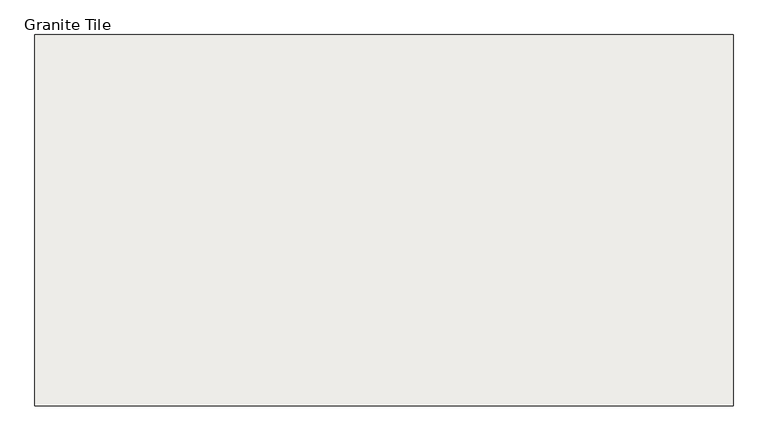
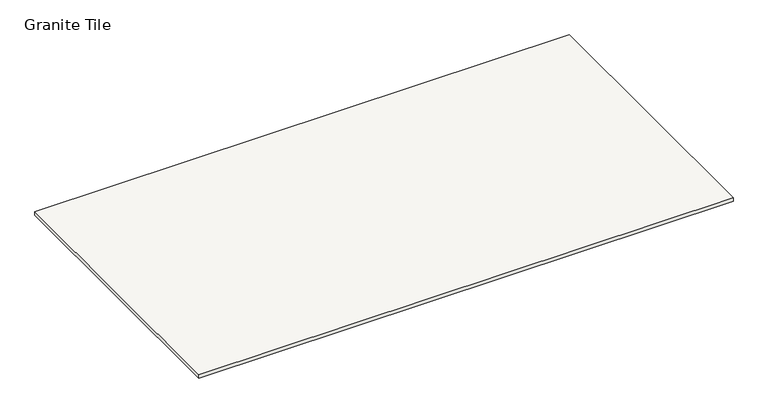
"""IFC4 building model written with IfcOpenShell, lengths in millimetres: slab geometry, Granite Tile."""

from ifc_helpers import new_model, si_unit, frame, origin, place, context, project, spatial, polyline, outline, extrude, source, transform, mapped, element, save


def granite_tile_fce40326(model_context):
    return source(origin(), model_context, "Body", "SweptSolid", [
        extrude(outline(polyline([(27200.0, 300.0), (22650.0, 300.0), (22650.0, 2720.0), (27200.0, 2720.0), (27200.0, 300.0)])), frame((0.0, 0.0, 4800.0), z_axis=(0.0, 0.0, 1.0), x_axis=(1.0, 0.0, 0.0)), (0.0, 0.0, 1.0), 30.0),
    ])


if __name__ == "__main__":
    model = new_model("IFC4")
    model_context = context("Model", 3, world=origin())
    ifc_project = project(units=[si_unit("LENGTHUNIT", "METRE", prefix="MILLI")], contexts=[model_context])
    site = spatial("IfcSite", under=ifc_project)
    building = spatial("IfcBuilding", under=site)
    placement = place(None, origin())
    granite_tile_shape = granite_tile_fce40326(model_context)
    element("IfcSlab", 1, ObjectType="Granite Tile", at=placement, inside=building, context=model_context, shape_type="MappedRepresentation", body=[
        mapped(granite_tile_shape, transform((0.0, 0.0, 0.0), x_axis=(1.0, 0.0, 0.0), y_axis=(0.0, 1.0, 0.0), z_axis=(0.0, 0.0, 1.0))),
    ])
    save(model, "model.ifc")

# Revit data of these elements
# Element 1 (IfcSlab, "Granite Tile")
#   Materials on its faces: "00_Stone_Granite"
# Materials
#   "00_Stone_Granite": class "Stone", colour RGB 99 103 98, transparency 0, Description = "Granite", Cost = 0, Image = Masonry.Stone.Granite.Square.Stacked.Polished.Black-White.jpg
